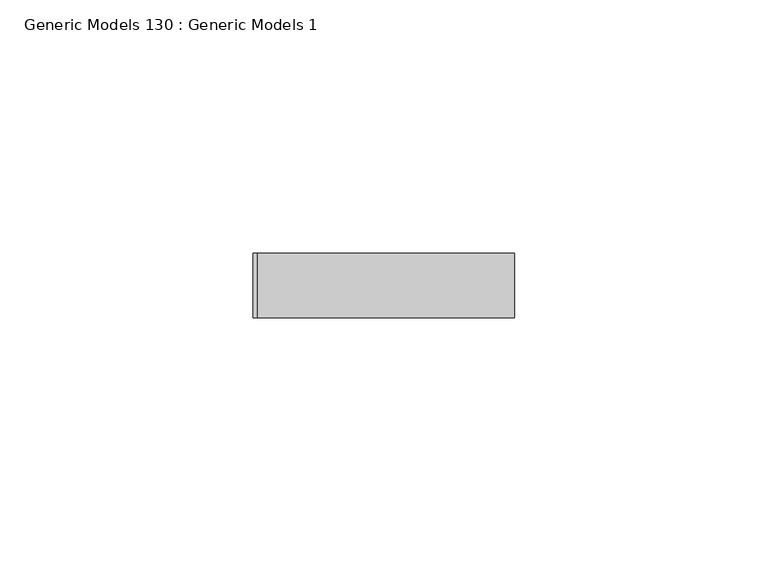
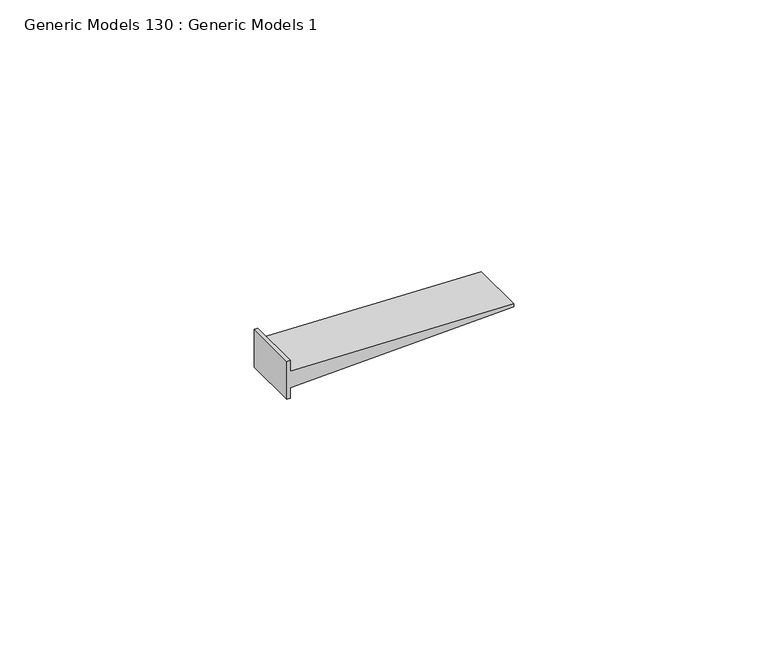
"""IFC4 building model written with IfcOpenShell, lengths in millimetres: proxy geometry, Generic Models 130 : Generic Models 1."""

from ifc_helpers import new_model, si_unit, frame, origin, place, context, project, spatial, polyline, outline, extrude, source, transform, mapped, element, save


def generic_models_130_generic_models_1_00598c4c(model_context):
    return source(origin(), model_context, "Body", "SweptSolid", [
        extrude(outline(polyline([(259.1857124, 49693.5744139), (250.0925124, 49693.5744139), (250.0925124, 49694.3681639), (252.642376, 49694.3681639), (254.2397651, 49745.1681639), (255.0384597, 49745.1681639), (256.6358488, 49694.3681639), (259.1857124, 49694.3681639), (259.1857124, 49693.5744139)])), frame((0.0, 565.15, 0.0), z_axis=(0.0, 1.0, 0.0), x_axis=(0.0, 0.0, 1.0)), (0.0, 0.0, 1.0), 12.7),
    ])


if __name__ == "__main__":
    model = new_model("IFC4")
    model_context = context("Model", 3, world=origin())
    ifc_project = project(units=[si_unit("LENGTHUNIT", "METRE", prefix="MILLI")], contexts=[model_context])
    site = spatial("IfcSite", under=ifc_project)
    building = spatial("IfcBuilding", under=site)
    placement = place(None, origin())
    generic_models_130_generic_models_1_shape = generic_models_130_generic_models_1_00598c4c(model_context)
    element("IfcBuildingElementProxy", 1, Name="Generic Models 130 : Generic Models 1", ObjectType="Generic Models 130 : Generic Models 1", at=placement, inside=building, context=model_context, shape_type="MappedRepresentation", body=[
        mapped(generic_models_130_generic_models_1_shape, transform((0.0, 0.0, 0.0), x_axis=(1.0, 0.0, 0.0), y_axis=(0.0, 1.0, 0.0), z_axis=(0.0, 0.0, 1.0))),
    ])
    save(model, "model.ifc")

# Revit data of these elements
# Project information
#   Project Issue Date = "09.19.2018"
#   Project Status = "Project Status"
#   Client Name = "Owner"
#   Project Address = "4519 MONONA DR, MONONA, WI 53716"
#   Project Name = "SPRINGHAVEN LAUNDRY"
#   Project Number = "Project Number"
# Element 1 (IfcBuildingElementProxy, "Generic Models 130 : Generic Models 1")
#   Materials on its faces: "ATTACH GYPSUM BOARD TO STUDS AND NOT TO TOP TRACK"
# Materials
#   "ATTACH GYPSUM BOARD TO STUDS AND NOT TO TOP TRACK": class "Generic", colour RGB 48 48 48, transparency 0, Cost = 0
